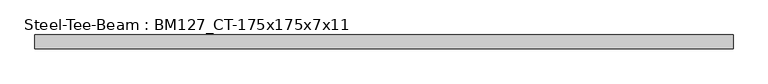
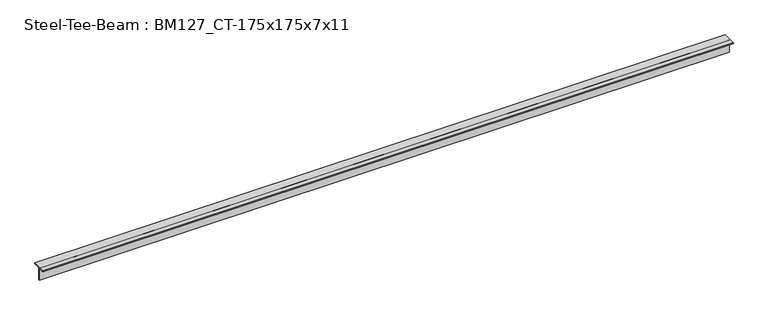
"""IFC4 building model written with IfcOpenShell, lengths in millimetres: beam geometry, Steel-Tee-Beam : BM127_CT-175x175x7x11."""

from ifc_helpers import new_model, si_unit, point, frame, frame_2d, origin, place, context, project, spatial, polyline, circle_curve, trimmed, segment, composite_curve, outline, extrude, source, transform, mapped, element, save


def steel_tee_beam_bm127_ct_175x175x7x11_6c364353(model_context):
    return source(origin(), model_context, "Body", "SweptSolid", [
        extrude(outline(composite_curve([segment(polyline([(-87.5, 87.5), (87.5, 87.5), (87.5, 76.5), (17.5, 76.5)]), True, "CONTINUOUS"), segment(trimmed(circle_curve(frame_2d((17.5, 62.5)), 14.0), [point((17.5, 76.5))], [point((3.5, 62.5))], True, "CARTESIAN"), True, "CONTINUOUS"), segment(polyline([(3.5, 62.5), (3.5, -87.5), (-3.5, -87.5), (-3.5, 62.5)]), True, "CONTINUOUS"), segment(trimmed(circle_curve(frame_2d((-17.5, 62.5)), 14.0), [point((-3.5, 62.5))], [point((-17.5, 76.5))], True, "CARTESIAN"), True, "CONTINUOUS"), segment(polyline([(-17.5, 76.5), (-87.5, 76.5), (-87.5, 87.5)]), True, "CONTINUOUS")], self_intersect=False)), frame((-4427.0238227, 0.0, 0.0), z_axis=(1.0, 0.0, 0.0), x_axis=(0.0, 1.0, 0.0)), (0.0, 0.0, 1.0), 8723.5825238),
    ])


if __name__ == "__main__":
    model = new_model("IFC4")
    model_context = context("Model", 3, world=origin())
    ifc_project = project(units=[si_unit("LENGTHUNIT", "METRE", prefix="MILLI")], contexts=[model_context])
    site = spatial("IfcSite", under=ifc_project)
    building = spatial("IfcBuilding", under=site)
    placement = place(None, origin())
    steel_tee_beam_bm127_ct_175x175x7x11_shape = steel_tee_beam_bm127_ct_175x175x7x11_6c364353(model_context)
    element("IfcBeam", 1, ObjectType="Steel-Tee-Beam : BM127_CT-175x175x7x11", at=placement, inside=building, context=model_context, shape_type="MappedRepresentation", body=[
        mapped(steel_tee_beam_bm127_ct_175x175x7x11_shape, transform((0.0, 0.0, 0.0), x_axis=(1.0, 0.0, 0.0), y_axis=(0.0, 1.0, 0.0), z_axis=(0.0, 0.0, 1.0))),
    ])
    save(model, "model.ifc")

# Revit data of these elements
# Type "Steel-Tee-Beam : BM127_CT-175x175x7x11"
#   Surface Area = 0.00 m²/m
#   Section Area = 31.57 cm²
#   Mass per Unit Length = 24.80 kg/m
#   Length [instance default] = 1524 mm
#   bf = 175 mm
#   d = 175 mm
#   k = 25 mm
#   kr = 14 mm
#   tf = 11 mm
#   tw = 7 mm
#   hec_material4 [instance default] = none
#   hec_material3 [instance default] = none
#   hec_material2 [instance default] = none
#   hec_material1 [instance default] = none
#   Structural Material [instance default] = Steel, 45-345
#   Assembly Code = ""
# Element 1 (IfcBeam, "Steel-Tee-Beam : BM127_CT-175x175x7x11")
#   hec_material3 = F01AC000-00002_Building/Shelter Fire Proofing Work_Intumescent Coating Type_1 hr. rating (UL 1709))
#   hec_material2 = S01AA010-00002_Main Steel Structure Fabrication Work_Shelter/Building_Steel Painting/Coating_for Fireproofed Steel Surface, Surface Preparation & Primer Coat
#   hec_material1 = S03AA029-00001_Main Steel Structure Erection Work_Shelter/Building_Light Steel
#   Structural Material = S01AA003-00001_Main Steel Structure Fabrication Work_Shelter/Building_Light Steel - Standard
#   Materials on its faces: "S01AA003-00001_Main Steel Structure Fabrication Work_Shelter/Building_Light Steel - Standard"
# Materials
#   "Steel, 45-345": class "Metal", colour RGB 189 187 185, transparency 0, Description = "Steel 345 MPa", Cost = 0
#   "S01AA003-00001_Main Steel Structure Fabrication Work_Shelter/Building_Light Steel - Standard": class "Metal", colour RGB 120 120 120, transparency 0, Comments = "(30KG/M>Weight)", Description = "Structural steel 50ksi", W00) Work Master Code = "S01AA003-00001", W01) Work Master_Lv1 = "Main Steel Structure Fabrication Work", W02) Work Master_Lv2 = "Shelter/Building", W03) Work Master_Spec.1 = "Light Steel - Standard (30KG/M>Weight)", Cost = 0
#   "F01AC000-00002_Building/Shelter Fire Proofing Work_Intumescent Coating Type_1 hr. rating (UL 1709))": class "Metal", colour RGB 255 128 128, transparency 0, Description = "Paint finished steel", W00) Work Master Code = "F01AC000-00002", W01) Work Master_Lv1 = "Building/Shelter Fire Proofing Work", W02) Work Master_Lv2 = "Intumescent Coating Type", W03) Work Master_Spec.1 = "1 hr. rating (UL 1709)", Cost = 0
#   "S01AA010-00002_Main Steel Structure Fabrication Work_Shelter/Building_Steel Painting/Coating_for Fireproofed Steel Surface, Surface Preparation & Primer Coat": class "Metal", colour RGB 120 120 120, transparency 0, Description = "Paint finished steel", W00) Work Master Code = "SS01AA010-00002", W01) Work Master_Lv1 = "Main Steel Structure Fabrication Work", W02) Work Master_Lv2 = "Shelter/Building", W03) Work Master_Spec.1 = "Steel Painting/Coating", W04) Work Master_Spec.2 = "for Fireproofed Steel Surface, Surface Preparation & Primer Coat", Cost = 0
#   "S03AA029-00001_Main Steel Structure Erection Work_Shelter/Building_Light Steel": class "Metal", colour RGB 120 120 120, transparency 0, Comments = "(30KG/M>Weight)", Description = "Structural steel 50ksi", W00) Work Master Code = "S03AA029-00001", W01) Work Master_Lv1 = "Main Steel Structure Erection Work", W02) Work Master_Lv2 = "Shelter/Building", W03) Work Master_Spec.1 = "Light Steel (30KG/M>Weight)", Cost = 0
